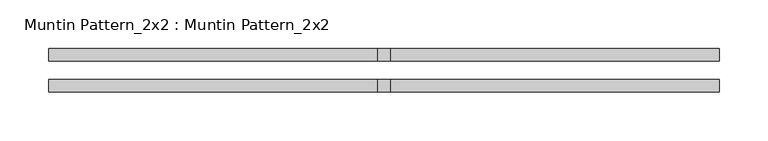
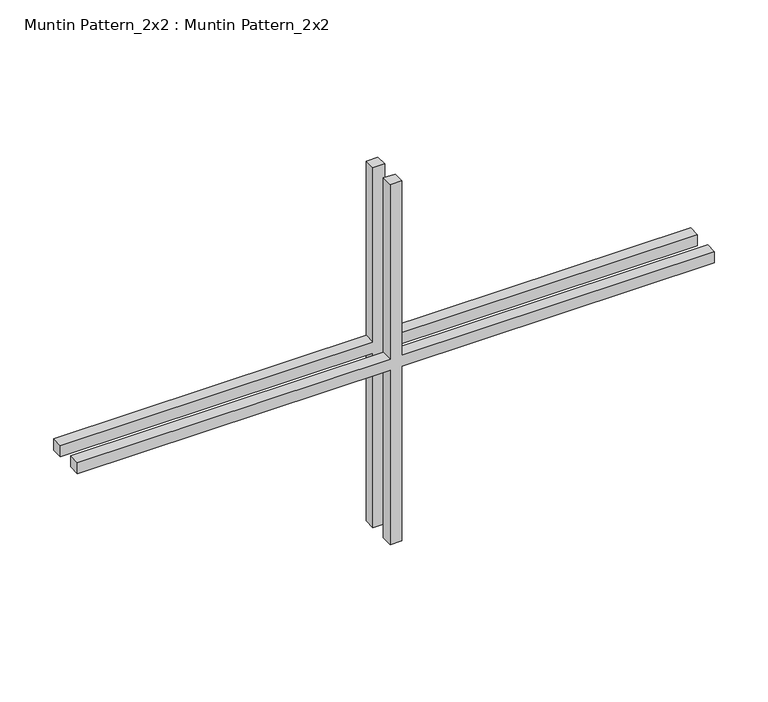
"""IFC4 building model written with IfcOpenShell, lengths in millimetres: proxy geometry, Muntin Pattern_2x2 : Muntin Pattern_2x2."""

from ifc_helpers import new_model, si_unit, frame, origin, place, context, project, spatial, polyline, outline, extrude, source, transform, mapped, element, save


def muntin_pattern_2x2_muntin_pattern_2x2_f86c9fba(model_context):
    return source(origin(), model_context, "Body", "SweptSolid", [
        extrude(outline(polyline([(211.1375, -6.35), (211.1375, -342.9), (198.4375, -342.9), (198.4375, -6.35), (0.0, -6.35), (0.0, 6.35), (198.4375, 6.35), (198.4375, 342.9), (211.1375, 342.9), (211.1375, 6.35), (409.575, 6.35), (409.575, -6.35), (211.1375, -6.35)])), frame((0.0, -22.225, 0.0), z_axis=(0.0, 1.0, 0.0), x_axis=(0.0, 0.0, 1.0)), (0.0, 0.0, 1.0), 12.7),
        extrude(outline(polyline([(211.1375, -6.35), (211.1375, -342.9), (198.4375, -342.9), (198.4375, -6.35), (0.0, -6.35), (0.0, 6.35), (198.4375, 6.35), (198.4375, 342.9), (211.1375, 342.9), (211.1375, 6.35), (409.575, 6.35), (409.575, -6.35), (211.1375, -6.35)])), frame((0.0, 9.525, 0.0), z_axis=(0.0, 1.0, 0.0), x_axis=(0.0, 0.0, 1.0)), (0.0, 0.0, 1.0), 12.7),
    ])


if __name__ == "__main__":
    model = new_model("IFC4")
    model_context = context("Model", 3, world=origin())
    ifc_project = project(units=[si_unit("LENGTHUNIT", "METRE", prefix="MILLI")], contexts=[model_context])
    site = spatial("IfcSite", under=ifc_project)
    building = spatial("IfcBuilding", under=site)
    placement = place(None, origin())
    muntin_pattern_2x2_muntin_pattern_2x2_shape = muntin_pattern_2x2_muntin_pattern_2x2_f86c9fba(model_context)
    element("IfcBuildingElementProxy", 1, Name="Muntin Pattern_2x2 : Muntin Pattern_2x2", ObjectType="Muntin Pattern_2x2 : Muntin Pattern_2x2", at=placement, inside=building, context=model_context, shape_type="MappedRepresentation", body=[
        mapped(muntin_pattern_2x2_muntin_pattern_2x2_shape, transform((0.0, 0.0, 0.0), x_axis=(1.0, 0.0, 0.0), y_axis=(0.0, 1.0, 0.0), z_axis=(0.0, 0.0, 1.0))),
    ])
    save(model, "model.ifc")

# Revit data of these elements
# Type "Muntin Pattern_2x2 : Muntin Pattern_2x2"
#   Width [instance default] = 4' - 0"
#   Thickness = 0' - 0 1/2"
#   Height [instance default] = 4' - 0"
#   Distance = 0' - 0 3/4"
#   Interior Material [instance default] = none
#   Exterior Material [instance default] = none
# Element 1 (IfcBuildingElementProxy, "Muntin Pattern_2x2 : Muntin Pattern_2x2")
#   Width = 2' - 3"
#   Height = 1' - 4 1/8"
#   Interior Material = Wood - Stained
#   Exterior Material = Clad - White
#   Materials on its faces: "Clad - White", "Wood - Stained"
# Materials
#   "Clad - White": class "Wood", colour RGB 242 242 238, transparency 0, Cost = 0
#   "Wood - Stained": class "Wood", colour RGB 224 178 126, transparency 0, Cost = 0
